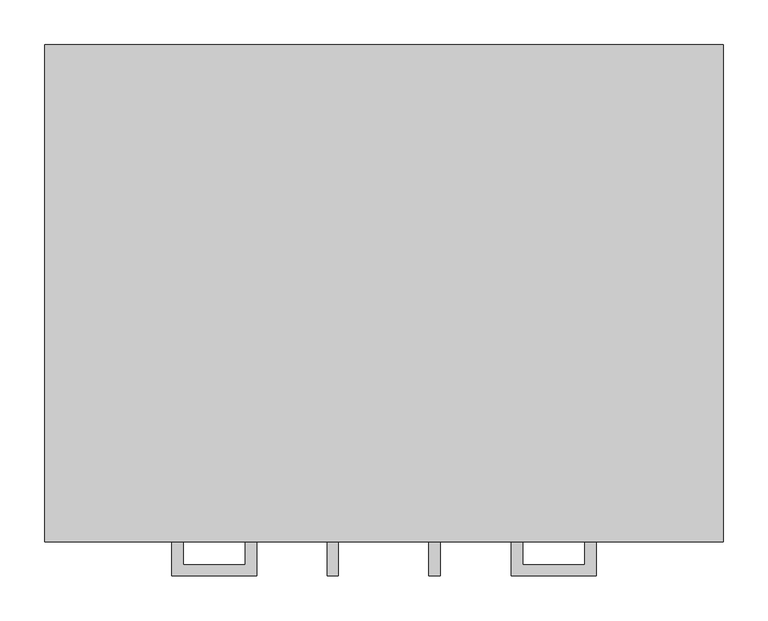
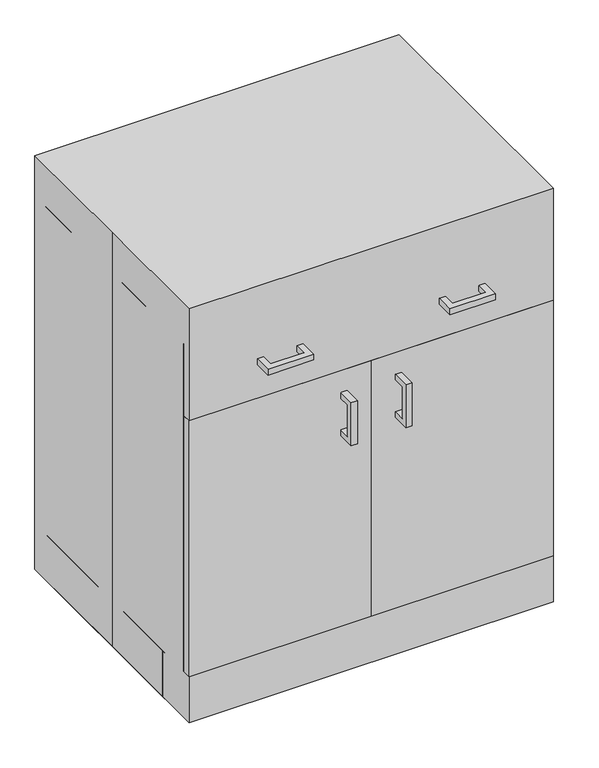
"""IFC4 building model written with IfcOpenShell, lengths in millimetres: proxy geometry, C03F0 - Cabinet, U-C-B, 1 Shelf, 2 Half DR, 2 DO, 36x30x22 : C03F0 - Cabinet, U-C-B, 1 Shelf, 2 Half DR, 2 DO, 36x30x22."""

from ifc_helpers import new_model, si_unit, frame, origin, origin_with_axes, place, context, project, spatial, polyline, outline, extrude, source, transform, mapped, element, save


def specialty_equipment_70df37de(model_context):
    return source(origin(), model_context, "Body", "SweptSolid", [
        extrude(outline(polyline([(0.0, -279.4), (-381.0, -279.4), (-381.0, -260.35), (0.0, -260.35), (0.0, -279.4)])), frame((0.0, 0.0, 101.6), z_axis=(0.0, 0.0, 1.0), x_axis=(1.0, 0.0, 0.0)), (0.0, 0.0, 1.0), 565.15),
        extrude(outline(polyline([(-238.125, -317.5), (-238.125, -279.4), (-225.4409299, -279.4), (-225.4409299, -304.8159299), (-155.5590701, -304.8159299), (-155.5590701, -279.4), (-142.875, -279.4), (-142.875, -317.5), (-238.125, -317.5)])), frame((0.0, 0.0, 741.3462383), z_axis=(0.0, 0.0, 1.0), x_axis=(1.0, 0.0, 0.0)), (0.0, 0.0, 1.0), 12.7),
        extrude(outline(polyline([(238.125, -317.5), (142.875, -317.5), (142.875, -279.4), (155.5590701, -279.4), (155.5590701, -304.8159299), (225.4409299, -304.8159299), (225.4409299, -279.4), (238.125, -279.4), (238.125, -317.5)])), frame((0.0, 0.0, 741.3462383), z_axis=(0.0, 0.0, 1.0), x_axis=(1.0, 0.0, 0.0)), (0.0, 0.0, 1.0), 12.7),
        extrude(outline(polyline([(381.0, -279.4), (0.0, -279.4), (0.0, -260.35), (381.0, -260.35), (381.0, -279.4)])), frame((0.0, 0.0, 101.6), z_axis=(0.0, 0.0, 1.0), x_axis=(1.0, 0.0, 0.0)), (0.0, 0.0, 1.0), 565.15),
        extrude(outline(polyline([(-317.5, 523.8560937), (-317.5, 619.1060937), (-279.4, 619.1060937), (-279.4, 606.4220236), (-304.8159299, 606.4220236), (-304.8159299, 536.5401637), (-279.4, 536.5401637), (-279.4, 523.8560937), (-317.5, 523.8560937)])), frame((50.5065288, 0.0, 0.0), z_axis=(1.0, 0.0, 0.0), x_axis=(0.0, 1.0, 0.0)), (0.0, 0.0, 1.0), 12.7),
        extrude(outline(polyline([(-317.5, 523.8560937), (-317.5, 619.1060937), (-279.4, 619.1060937), (-279.4, 606.4220236), (-304.8159299, 606.4220236), (-304.8159299, 536.5401637), (-279.4, 536.5401637), (-279.4, 523.8560937), (-317.5, 523.8560937)])), frame((-63.7934712, 0.0, 0.0), z_axis=(1.0, 0.0, 0.0), x_axis=(0.0, 1.0, 0.0)), (0.0, 0.0, 1.0), 12.7),
        extrude(outline(polyline([(-381.0, 279.4), (381.0, 279.4), (381.0, -279.4), (-381.0, -279.4), (-381.0, 0.0), (-381.0, 279.4)])), origin_with_axes(), (0.0, 0.0, 1.0), 914.4),
        extrude(outline(polyline([(381.0, -279.4), (0.0, -279.4), (0.0, -260.35), (381.0, -260.35), (381.0, -279.4)])), frame((0.0, 0.0, 673.0674767), z_axis=(0.0, 0.0, 1.0), x_axis=(1.0, 0.0, 0.0)), (0.0, 0.0, 1.0), 152.4),
        extrude(outline(polyline([(0.0, -279.4), (-381.0, -279.4), (-381.0, -260.35), (0.0, -260.35), (0.0, -279.4)])), frame((0.0, 0.0, 673.0674767), z_axis=(0.0, 0.0, 1.0), x_axis=(1.0, 0.0, 0.0)), (0.0, 0.0, 1.0), 152.4),
        extrude(outline(polyline([(-381.0, -260.35), (-381.0, 279.4), (-361.95, 279.4), (-361.95, -260.35), (-381.0, -260.35)])), frame((0.0, 0.0, 101.6), z_axis=(0.0, 0.0, 1.0), x_axis=(1.0, 0.0, 0.0)), (0.0, 0.0, 1.0), 723.8674767),
        extrude(outline(polyline([(361.95, -260.35), (361.95, 279.4), (381.0, 279.4), (381.0, -260.35), (361.95, -260.35)])), frame((0.0, 0.0, 101.6), z_axis=(0.0, 0.0, 1.0), x_axis=(1.0, 0.0, 0.0)), (0.0, 0.0, 1.0), 723.8674767),
        extrude(outline(polyline([(381.0, -203.2), (-381.0, -203.2), (-381.0, -184.15), (381.0, -184.15), (381.0, -203.2)])), origin_with_axes(), (0.0, 0.0, 1.0), 101.6),
        extrude(outline(polyline([(-381.0, -184.15), (-381.0, 279.4), (-361.95, 279.4), (-361.95, -184.15), (-381.0, -184.15)])), origin_with_axes(), (0.0, 0.0, 1.0), 101.6),
        extrude(outline(polyline([(361.95, -184.15), (361.95, 279.4), (381.0, 279.4), (381.0, -184.15), (361.95, -184.15)])), origin_with_axes(), (0.0, 0.0, 1.0), 101.6),
        extrude(outline(polyline([(381.0, 260.35), (-381.0, 260.35), (-381.0, 279.4), (381.0, 279.4), (381.0, 260.35)])), origin_with_axes(), (0.0, 0.0, 1.0), 101.6),
        extrude(outline(polyline([(361.95, 260.35), (361.95, -260.35), (-361.95, -260.35), (-361.95, 260.35), (361.95, 260.35)])), frame((0.0, 0.0, 101.6), z_axis=(0.0, 0.0, 1.0), x_axis=(1.0, 0.0, 0.0)), (0.0, 0.0, 1.0), 19.1166954),
        extrude(outline(polyline([(361.95, 260.35), (-361.95, 260.35), (-361.95, 279.4), (361.95, 279.4), (361.95, 260.35)])), frame((0.0, 0.0, 101.6), z_axis=(0.0, 0.0, 1.0), x_axis=(1.0, 0.0, 0.0)), (0.0, 0.0, 1.0), 704.8174767),
    ])


if __name__ == "__main__":
    model = new_model("IFC4")
    model_context = context("Model", 3, world=origin())
    ifc_project = project(units=[si_unit("LENGTHUNIT", "METRE", prefix="MILLI")], contexts=[model_context])
    site = spatial("IfcSite", under=ifc_project)
    building = spatial("IfcBuilding", under=site)
    placement = place(None, origin())
    specialty_equipment_shape = specialty_equipment_70df37de(model_context)
    element("IfcBuildingElementProxy", 1, Name="C03F0 - Cabinet, U-C-B, 1 Shelf, 2 Half DR, 2 DO, 36x30x22 : C03F0 - Cabinet, U-C-B, 1 Shelf, 2 Half DR, 2 DO, 36x30x22", ObjectType="C03F0 - Cabinet, U-C-B, 1 Shelf, 2 Half DR, 2 DO, 36x30x22 : C03F0 - Cabinet, U-C-B, 1 Shelf, 2 Half DR, 2 DO, 36x30x22", at=placement, inside=building, context=model_context, shape_type="MappedRepresentation", body=[
        mapped(specialty_equipment_shape, transform((0.0, 0.0, 0.0), x_axis=(1.0, 0.0, 0.0), y_axis=(0.0, 1.0, 0.0), z_axis=(0.0, 0.0, 1.0))),
    ])
    save(model, "model.ifc")

# Revit data of these elements
# Project information
#   Room Abbreviation = "XDUS1/TLTU1"
#   Room Description 2-1 = "Xray, Ultrasound (XDUS1)"
#   Room Description 2-2 = "Toilet, (TLTU1)"
#   Sheets - Total = "6"
#   Project Issue Date = "Issue Date"
#   Project Status = "Project Status"
#   Client Name = "Owner"
#   Project Address = "Enter address here"
#   Project Name = "Project Name"
#   Project Number = "Project Number"
#   Publication Date = "30-Jan-15"
# Type "C03F0 - Cabinet, U-C-B, 1 Shelf, 2 Half DR, 2 DO, 36x30x22 : C03F0 - Cabinet, U-C-B, 1 Shelf, 2 Half DR, 2 DO, 36x30x22"
#   Watts2 = "0"
#   Watts1 = "0"
#   Unit_Issue = "EA"
#   UTIL_6_Misc = "-"
#   UTIL_5_NonMedGas = "-"
#   UTIL_4_MiscGas = "-"
#   UTIL_3_MedGas = "-"
#   UTIL_2_Elec = "-"
#   UTIL_1_WaterDrain = "-"
#   Nomenclature = "Cabinet, U/C/B, 1 Shelf, 2 Half DR, 2 DO, 36x30x22"
#   NSN = "6530"
#   Location [instance default] = ""
#   JSN = "C03F0"
#   Fund_Source_VA = "-"
#   Fund_Source_Navy = "-"
#   Fund_Source_Army = "-"
#   Fund_Source_AF = "-"
#   ELEC_Volts2 = "0"
#   ELEC_Volts1 = "0"
#   ELEC_Phase2 = "0"
#   ELEC_Phase1 = "0"
#   ELEC_HertzSwitch = "0"
#   ELEC_HertzDependent = "0"
#   ELEC_Hertz = "0"
#   ELEC_Amps2 = "0"
#   ELEC_Amps1 = "0"
#   DetailDescription = "Standing height under counter base cabinet with an adjustable shelf and two half width drawers above solid hinged doors. Also referred to as a combination cabinet or a drawer and cupboard cabinet. For general purpose use throughout the facility."
#   CAT_VA = "A"
#   CAT_Navy = "A"
#   CAT_IHS = "-"
#   CAT_Army = "A"
#   CAT_AF = "A"
#   BTUperhour = "0"
#   Weight_IP = 130
#   DIM_Width_IP = 2' - 6"
#   DIM_Height_IP = 3' - 0"
#   DIM_Depth_IP = 1' - 10"
#   Top Panel Material = none
#   Toe Panel Material = none
#   Side Panel Material = none
#   Shelf Panel Material = none
#   Drawer Front Material = none
#   Door Panel Material = none
#   Back Panel Material = none
#   Assembly Code = ""
# Element 1 (IfcBuildingElementProxy, "C03F0 - Cabinet, U-C-B, 1 Shelf, 2 Half DR, 2 DO, 36x30x22 : C03F0 - Cabinet, U-C-B, 1 Shelf, 2 Half DR, 2 DO, 36x30x22")
#   Location = "XDUS1"
#   Materials on its faces: "Default metal", "EquipSpace"
# Materials
#   "Default metal": class "Unassigned", colour RGB 204 204 204, transparency 0
#   "EquipSpace": class "Unassigned", colour RGB 221 217 195, transparency 0.5
